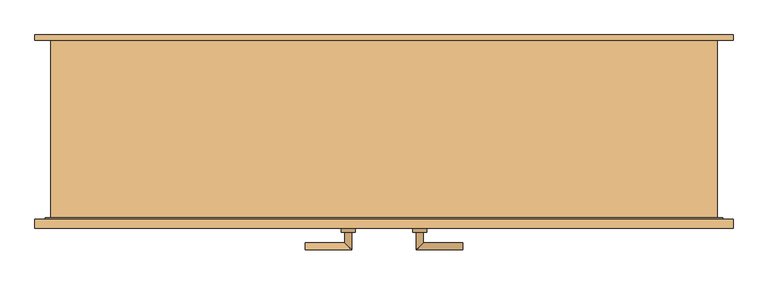
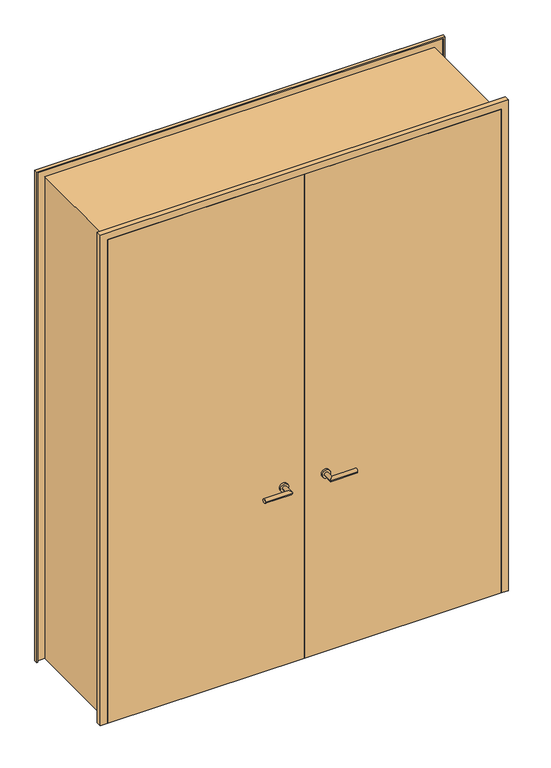
"""IFC4 building model written with IfcOpenShell, lengths in millimetres: door geometry, Drehflügel 2-flg - Stahlzarge : Holztüre 2 flg.1.9x 2.45."""

from ifc_helpers import new_model, si_unit, point, frame, frame_2d, origin, place, context, project, spatial, polyline, circle_curve, ellipse_curve, trimmed, segment, composite_curve, outline, extrude, faceted_brep, source, transform, mapped, element, save
from ifc_brep_helpers import plane_surface, cylinder_surface, advanced_brep


def door_26f10a8e(model_context):
    return source(origin(), model_context, "Body", "SolidModel", [
        advanced_brep(
        [(-90.0, -239.4346141, 1000.0), (-110.0, -239.4346141, 1000.0), (-90.0, -169.4346141, 1000.0), (-110.0, -189.4346141, 1000.0), (-220.0, -169.4346141, 1000.0), (-220.0, -189.4346141, 1000.0)],
        [
            (0, 1, circle_curve(frame((-100.0, -239.4346141, 1000.0), z_axis=(0.0, -1.0, 0.0), x_axis=(-1.0, 0.0, 0.0)), 10.0)),
            (1, 0, circle_curve(frame((-100.0, -239.4346141, 1000.0), z_axis=(0.0, -1.0, 0.0), x_axis=(-1.0, 0.0, 0.0)), 10.0)),
            (0, 2),
            (2, 3, ellipse_curve(frame((-100.0, -179.4346141, 1000.0), z_axis=(0.7071067811865385, -0.7071067811865565, 0.0), x_axis=(-0.7071067811865563, -0.7071067811865386, 0.0)), 14.1421356, 10.0)),
            (3, 1),
            (3, 2, ellipse_curve(frame((-100.0, -179.4346141, 1000.0), z_axis=(0.7071067811865385, -0.7071067811865565, 0.0), x_axis=(-0.7071067811865563, -0.7071067811865386, 0.0)), 14.1421356, 10.0)),
            (4, 5, circle_curve(frame((-220.0, -179.4346141, 1000.0), z_axis=(-1.0, 0.0, 0.0), x_axis=(0.0, -1.0, 0.0)), 10.0)),
            (5, 4, circle_curve(frame((-220.0, -179.4346141, 1000.0), z_axis=(-1.0, 0.0, 0.0), x_axis=(0.0, -1.0, 0.0)), 10.0)),
            (2, 4),
            (5, 3),
        ],
        [
            plane_surface(frame((-100.0, -239.4346141, -287.7526403), z_axis=(0.0, -1.0, 0.0), x_axis=(0.0, 0.0, 1.0))),
            cylinder_surface(frame((-100.0, -239.4346141, 1000.0), z_axis=(0.0, -1.0, 0.0), x_axis=(-1.0, 0.0, 0.0)), 10.0),
            plane_surface(frame((-220.0, -179.4346141, -287.7526403), z_axis=(-1.0, 0.0, 0.0), x_axis=(0.0, 0.0, 1.0))),
            cylinder_surface(frame((-100.0, -179.4346141, 1000.0), z_axis=(1.0, 0.0, 0.0), x_axis=(0.0, -1.0, 0.0)), 10.0),
        ],
        [
            (0, [[1, 2]]),
            (1, [[-1, 3, 4, 5]]),
            (1, [[-2, -5, 6, -3]]),
            (2, [[7, 8]]),
            (3, [[-4, 9, -8, 10]]),
            (3, [[-6, -10, -7, -9]]),
        ],
    ),
        advanced_brep(
        [(-110.0, -299.4346141, 1000.0), (-90.0, -299.4346141, 1000.0), (-110.0, -329.4346141, 1000.0), (-90.0, -349.4346141, 1000.0), (-220.0, -329.4346141, 1000.0), (-220.0, -349.4346141, 1000.0)],
        [
            (0, 1, circle_curve(frame((-100.0, -299.4346141, 1000.0), z_axis=(0.0, 1.0, 0.0), x_axis=(1.0, 0.0, 0.0)), 10.0)),
            (1, 0, circle_curve(frame((-100.0, -299.4346141, 1000.0), z_axis=(0.0, 1.0, 0.0), x_axis=(1.0, 0.0, 0.0)), 10.0)),
            (0, 2),
            (2, 3, ellipse_curve(frame((-100.0, -339.4346141, 1000.0), z_axis=(0.7071067811865475, 0.7071067811865475, 0.0), x_axis=(-0.7071067811865474, 0.7071067811865476, 0.0)), 14.1421356, 10.0)),
            (3, 1),
            (3, 2, ellipse_curve(frame((-100.0, -339.4346141, 1000.0), z_axis=(0.7071067811865475, 0.7071067811865475, 0.0), x_axis=(-0.7071067811865474, 0.7071067811865476, 0.0)), 14.1421356, 10.0)),
            (4, 5, circle_curve(frame((-220.0, -339.4346141, 1000.0), z_axis=(-1.0, 0.0, 0.0), x_axis=(0.0, -1.0, 0.0)), 10.0)),
            (5, 4, circle_curve(frame((-220.0, -339.4346141, 1000.0), z_axis=(-1.0, 0.0, 0.0), x_axis=(0.0, -1.0, 0.0)), 10.0)),
            (2, 4),
            (5, 3),
        ],
        [
            plane_surface(frame((-100.0, -299.4346141, -287.7526403), z_axis=(0.0, 1.0, 0.0), x_axis=(0.0, 0.0, 1.0))),
            cylinder_surface(frame((-100.0, -299.4346141, 1000.0), z_axis=(0.0, 1.0, 0.0), x_axis=(1.0, 0.0, 0.0)), 10.0),
            plane_surface(frame((-220.0, -339.4346141, -287.7526403), z_axis=(-1.0, 0.0, 0.0), x_axis=(0.0, 0.0, 1.0))),
            cylinder_surface(frame((-100.0, -339.4346141, 1000.0), z_axis=(1.0, 0.0, 0.0), x_axis=(0.0, -1.0, 0.0)), 10.0),
        ],
        [
            (0, [[1, 2]]),
            (1, [[-1, 3, 4, 5]]),
            (1, [[-2, -5, 6, -3]]),
            (2, [[7, 8]]),
            (3, [[-4, 9, -8, 10]]),
            (3, [[-6, -10, -7, -9]]),
        ],
    ),
        extrude(outline(composite_curve([segment(trimmed(circle_curve(frame_2d((1000.0, -100.0)), 20.0), [point((1000.0, -80.0))], [point((1000.0, -120.0))], False, "CARTESIAN"), True, "CONTINUOUS"), segment(trimmed(circle_curve(frame_2d((1000.0, -100.0)), 20.0), [point((1000.0, -120.0))], [point((1000.0, -80.0))], False, "CARTESIAN"), True, "CONTINUOUS")], self_intersect=False)), frame((0.0, -239.4346141, 0.0), z_axis=(0.0, 1.0, 0.0), x_axis=(0.0, 0.0, 1.0)), (0.0, 0.0, 1.0), 10.0),
        extrude(outline(composite_curve([segment(trimmed(circle_curve(frame_2d((1000.0, -100.0)), 20.0), [point((1000.0, -80.0))], [point((1000.0, -120.0))], False, "CARTESIAN"), True, "CONTINUOUS"), segment(trimmed(circle_curve(frame_2d((1000.0, -100.0)), 20.0), [point((1000.0, -120.0))], [point((1000.0, -80.0))], False, "CARTESIAN"), True, "CONTINUOUS")], self_intersect=False)), frame((0.0, -299.4346141, 0.0), z_axis=(0.0, 1.0, 0.0), x_axis=(0.0, 0.0, 1.0)), (0.0, 0.0, 1.0), 10.0),
        advanced_brep(
        [(90.0, -239.4346141, 1000.0), (110.0, -239.4346141, 1000.0), (110.0, -189.4346141, 1000.0), (90.0, -169.4346141, 1000.0), (220.0, -169.4346141, 1000.0), (220.0, -189.4346141, 1000.0)],
        [
            (0, 1, circle_curve(frame((100.0, -239.4346141, 1000.0), z_axis=(0.0, -1.0, 0.0), x_axis=(1.0, 0.0, 0.0)), 10.0)),
            (1, 0, circle_curve(frame((100.0, -239.4346141, 1000.0), z_axis=(0.0, -1.0, 0.0), x_axis=(1.0, 0.0, 0.0)), 10.0)),
            (1, 2),
            (2, 3, ellipse_curve(frame((100.0, -179.4346141, 1000.0), z_axis=(-0.7071067811865385, -0.7071067811865565, 0.0), x_axis=(0.7071067811865563, -0.7071067811865386, 0.0)), 14.1421356, 10.0)),
            (3, 0),
            (3, 2, ellipse_curve(frame((100.0, -179.4346141, 1000.0), z_axis=(-0.7071067811865385, -0.7071067811865565, 0.0), x_axis=(0.7071067811865563, -0.7071067811865386, 0.0)), 14.1421356, 10.0)),
            (4, 5, circle_curve(frame((220.0, -179.4346141, 1000.0), z_axis=(1.0, 0.0, 0.0), x_axis=(0.0, -1.0, 0.0)), 10.0)),
            (5, 4, circle_curve(frame((220.0, -179.4346141, 1000.0), z_axis=(1.0, 0.0, 0.0), x_axis=(0.0, -1.0, 0.0)), 10.0)),
            (2, 5),
            (4, 3),
        ],
        [
            plane_surface(frame((100.0, -239.4346141, -287.7526403), z_axis=(0.0, -1.0, 0.0), x_axis=(0.0, 0.0, 1.0))),
            cylinder_surface(frame((100.0, -239.4346141, 1000.0), z_axis=(0.0, -1.0, 0.0), x_axis=(1.0, 0.0, 0.0)), 10.0),
            plane_surface(frame((220.0, -179.4346141, -287.7526403), z_axis=(1.0, 0.0, 0.0), x_axis=(0.0, 0.0, 1.0))),
            cylinder_surface(frame((100.0, -179.4346141, 1000.0), z_axis=(-1.0, 0.0, 0.0), x_axis=(0.0, -1.0, 0.0)), 10.0),
        ],
        [
            (0, [[1, 2]]),
            (1, [[3, 4, 5, -2]]),
            (1, [[-5, 6, -3, -1]]),
            (2, [[7, 8]]),
            (3, [[9, -7, 10, -4]]),
            (3, [[-10, -8, -9, -6]]),
        ],
    ),
        advanced_brep(
        [(110.0, -299.4346141, 1000.0), (90.0, -299.4346141, 1000.0), (90.0, -349.4346141, 1000.0), (110.0, -329.4346141, 1000.0), (220.0, -329.4346141, 1000.0), (220.0, -349.4346141, 1000.0)],
        [
            (0, 1, circle_curve(frame((100.0, -299.4346141, 1000.0), z_axis=(0.0, 1.0, 0.0), x_axis=(-1.0, 0.0, 0.0)), 10.0)),
            (1, 0, circle_curve(frame((100.0, -299.4346141, 1000.0), z_axis=(0.0, 1.0, 0.0), x_axis=(-1.0, 0.0, 0.0)), 10.0)),
            (1, 2),
            (2, 3, ellipse_curve(frame((100.0, -339.4346141, 1000.0), z_axis=(-0.7071067811865475, 0.7071067811865475, 0.0), x_axis=(0.7071067811865474, 0.7071067811865476, 0.0)), 14.1421356, 10.0)),
            (3, 0),
            (3, 2, ellipse_curve(frame((100.0, -339.4346141, 1000.0), z_axis=(-0.7071067811865475, 0.7071067811865475, 0.0), x_axis=(0.7071067811865474, 0.7071067811865476, 0.0)), 14.1421356, 10.0)),
            (4, 5, circle_curve(frame((220.0, -339.4346141, 1000.0), z_axis=(1.0, 0.0, 0.0), x_axis=(0.0, -1.0, 0.0)), 10.0)),
            (5, 4, circle_curve(frame((220.0, -339.4346141, 1000.0), z_axis=(1.0, 0.0, 0.0), x_axis=(0.0, -1.0, 0.0)), 10.0)),
            (2, 5),
            (4, 3),
        ],
        [
            plane_surface(frame((100.0, -299.4346141, -287.7526403), z_axis=(0.0, 1.0, 0.0), x_axis=(0.0, 0.0, 1.0))),
            cylinder_surface(frame((100.0, -299.4346141, 1000.0), z_axis=(0.0, 1.0, 0.0), x_axis=(-1.0, 0.0, 0.0)), 10.0),
            plane_surface(frame((220.0, -339.4346141, -287.7526403), z_axis=(1.0, 0.0, 0.0), x_axis=(0.0, 0.0, 1.0))),
            cylinder_surface(frame((100.0, -339.4346141, 1000.0), z_axis=(-1.0, 0.0, 0.0), x_axis=(0.0, -1.0, 0.0)), 10.0),
        ],
        [
            (0, [[1, 2]]),
            (1, [[3, 4, 5, -2]]),
            (1, [[-5, 6, -3, -1]]),
            (2, [[7, 8]]),
            (3, [[9, -7, 10, -4]]),
            (3, [[-10, -8, -9, -6]]),
        ],
    ),
        extrude(outline(composite_curve([segment(trimmed(circle_curve(frame_2d((1000.0, 100.0)), 20.0), [point((1000.0, 80.0))], [point((1000.0, 120.0))], False, "CARTESIAN"), True, "CONTINUOUS"), segment(trimmed(circle_curve(frame_2d((1000.0, 100.0)), 20.0), [point((1000.0, 120.0))], [point((1000.0, 80.0))], False, "CARTESIAN"), True, "CONTINUOUS")], self_intersect=False)), frame((0.0, -239.4346141, 0.0), z_axis=(0.0, 1.0, 0.0), x_axis=(0.0, 0.0, 1.0)), (0.0, 0.0, 1.0), 10.0),
        extrude(outline(composite_curve([segment(trimmed(circle_curve(frame_2d((1000.0, 100.0)), 20.0), [point((1000.0, 80.0))], [point((1000.0, 120.0))], False, "CARTESIAN"), True, "CONTINUOUS"), segment(trimmed(circle_curve(frame_2d((1000.0, 100.0)), 20.0), [point((1000.0, 120.0))], [point((1000.0, 80.0))], False, "CARTESIAN"), True, "CONTINUOUS")], self_intersect=False)), frame((0.0, -299.4346141, 0.0), z_axis=(0.0, 1.0, 0.0), x_axis=(0.0, 0.0, 1.0)), (0.0, 0.0, 1.0), 10.0),
        extrude(outline(polyline([(0.0, -264.4346141), (0.0, -289.4346141), (-940.0, -289.4346141), (-940.0, -264.4346141), (0.0, -264.4346141)])), frame((0.0, 0.0, 100.0), z_axis=(0.0, 0.0, 1.0), x_axis=(1.0, 0.0, 0.0)), (0.0, 0.0, 1.0), 2440.0),
        extrude(outline(polyline([(940.0, -264.4346141), (940.0, -289.4346141), (0.0, -289.4346141), (0.0, -264.4346141), (940.0, -264.4346141)])), frame((0.0, 0.0, 100.0), z_axis=(0.0, 0.0, 1.0), x_axis=(1.0, 0.0, 0.0)), (0.0, 0.0, 1.0), 2440.0),
        faceted_brep([(974.5, 250.5653859, 100.0), (974.5, 235.5653859, 100.0), (969.5, 235.5653859, 100.0), (969.5, 245.5653859, 100.0), (930.0, 245.5653859, 100.0), (930.0, -259.4346141, 100.0), (945.0, -259.4346141, 100.0), (945.0, -284.4346141, 100.0), (969.5, -284.4346141, 100.0), (969.5, -264.4346141, 100.0), (974.5, -264.4346141, 100.0), (974.5, -289.4346141, 100.0), (940.0, -289.4346141, 100.0), (940.0, -264.4346141, 100.0), (925.0, -264.4346141, 100.0), (925.0, 250.5653859, 100.0), (925.0, 250.5653859, 2525.0), (-925.0, 250.5653859, 2525.0), (-925.0, 250.5653859, 100.0), (-974.5, 250.5653859, 100.0), (-974.5, 250.5653859, 2574.5), (974.5, 250.5653859, 2574.5), (925.0, -264.4346141, 2525.0), (940.0, -264.4346141, 2540.0), (-940.0, -264.4346141, 2540.0), (-940.0, -264.4346141, 100.0), (-925.0, -264.4346141, 100.0), (-925.0, -264.4346141, 2525.0), (940.0, -289.4346141, 2540.0), (974.5, -289.4346141, 2574.5), (-974.5, -289.4346141, 2574.5), (-974.5, -289.4346141, 100.0), (-940.0, -289.4346141, 100.0), (-940.0, -289.4346141, 2540.0), (974.5, -264.4346141, 2574.5), (969.5, -264.4346141, 2569.5), (-969.5, -264.4346141, 2569.5), (-969.5, -264.4346141, 100.0), (-974.5, -264.4346141, 100.0), (-974.5, -264.4346141, 2574.5), (969.5, -284.4346141, 2569.5), (945.0, -284.4346141, 2545.0), (-945.0, -284.4346141, 2545.0), (-945.0, -284.4346141, 100.0), (-969.5, -284.4346141, 100.0), (-969.5, -284.4346141, 2569.5), (945.0, -259.4346141, 2545.0), (930.0, -259.4346141, 2530.0), (-930.0, -259.4346141, 2530.0), (-930.0, -259.4346141, 100.0), (-945.0, -259.4346141, 100.0), (-945.0, -259.4346141, 2545.0), (930.0, 245.5653859, 2530.0), (969.5, 245.5653859, 2569.5), (-969.5, 245.5653859, 2569.5), (-969.5, 245.5653859, 100.0), (-930.0, 245.5653859, 100.0), (-930.0, 245.5653859, 2530.0), (969.5, 235.5653859, 2569.5), (974.5, 235.5653859, 2574.5), (-974.5, 235.5653859, 2574.5), (-974.5, 235.5653859, 100.0), (-969.5, 235.5653859, 100.0), (-969.5, 235.5653859, 2569.5)], [[[0, 1, 2, 3, 4, 5, 6, 7, 8, 9, 10, 11, 12, 13, 14, 15]], [[15, 16, 17, 18, 19, 20, 21, 0]], [[14, 22, 16, 15]], [[13, 23, 24, 25, 26, 27, 22, 14]], [[12, 28, 23, 13]], [[11, 29, 30, 31, 32, 33, 28, 12]], [[10, 34, 29, 11]], [[9, 35, 36, 37, 38, 39, 34, 10]], [[8, 40, 35, 9]], [[7, 41, 42, 43, 44, 45, 40, 8]], [[6, 46, 41, 7]], [[5, 47, 48, 49, 50, 51, 46, 6]], [[4, 52, 47, 5]], [[3, 53, 54, 55, 56, 57, 52, 4]], [[2, 58, 53, 3]], [[1, 59, 60, 61, 62, 63, 58, 2]], [[0, 21, 59, 1]], [[20, 19, 61, 60]], [[19, 18, 26, 25, 32, 31, 38, 37, 44, 43, 50, 49, 56, 55, 62, 61]], [[27, 26, 18, 17]], [[33, 32, 25, 24]], [[39, 38, 31, 30]], [[45, 44, 37, 36]], [[51, 50, 43, 42]], [[57, 56, 49, 48]], [[63, 62, 55, 54]], [[22, 27, 17, 16]], [[28, 33, 24, 23]], [[34, 39, 30, 29]], [[40, 45, 36, 35]], [[46, 51, 42, 41]], [[52, 57, 48, 47]], [[58, 63, 54, 53]], [[21, 20, 60, 59]]]),
    ])


if __name__ == "__main__":
    model = new_model("IFC4")
    model_context = context("Model", 3, world=origin())
    ifc_project = project(units=[si_unit("LENGTHUNIT", "METRE", prefix="MILLI")], contexts=[model_context])
    site = spatial("IfcSite", under=ifc_project)
    building = spatial("IfcBuilding", under=site)
    placement = place(None, origin())
    door_shape = door_26f10a8e(model_context)
    element("IfcDoor", 1, ObjectType="Drehflügel 2-flg - Stahlzarge : Holztüre 2 flg.1.9x 2.45", at=placement, inside=building, context=model_context, shape_type="MappedRepresentation", body=[
        mapped(door_shape, transform((0.0, 0.0, 0.0), x_axis=(1.0, 0.0, 0.0), y_axis=(0.0, 1.0, 0.0), z_axis=(0.0, 0.0, 1.0))),
    ])
    save(model, "model.ifc")

# Revit data of these elements
# Type "Drehflügel 2-flg - Stahlzarge : Holztüre 2 flg.1.9x 2.45"
#   Type Mark = "22"
#   Operation = "DoubleDoorSingleSwing"
#   Keynote = "16.03"
#   Analytic Construction = "Metall"
#   Thermal Resistance (R) = 0.270117 (m²·K)/W
#   Heat Transfer Coefficient (U) = 3.7021 W/(m²·K)
#   Rough Width = 1.900 m
#   Rough Height [instance default] = 2.550 m
#   Höhe Türgriff = 0.900 m
#   Height = 2.450 m
#   Fußbodenaufbau [instance default] = 0.100 m
#   Width = 1.900 m
#   Sichtbarkeit Sturzlinien [instance default] = yes
#   Türgriff auswählen [instance default] = element 219327
#   Türgriff [instance default] = none
#   Türflügel [instance default] = none
#   Rahmen/Pfosten [instance default] = Metall - Lackiert - Grau
#   Visual Light Transmittance = 0
#   Solar Heat Gain Coefficient = 0
#   Function = (empty or 0)
#   Wall Closure = (empty or 0)
# Element 1 (IfcDoor, "Drehflügel 2-flg - Stahlzarge : Holztüre 2 flg.1.9x 2.45")
#   Rahmen/Pfosten = Holz - Eiche
#   Materials on its faces: "Metall - Chrom", "Holz - Eiche", "Holz - Birke"
# Materials
#   "Metall - Lackiert - Grau": class "Farbe 1", colour RGB 98 98 98, transparency 0, Cost = 0
#   "Metall - Chrom": class "Metall", colour RGB 247 247 247, transparency 0, Cost = 0
#   "Holz - Eiche": class "Holz", colour RGB 151 89 53, transparency 0, Cost = 0
#   "Holz - Birke": class "Holz", colour RGB 213 164 103, transparency 0, Cost = 0
